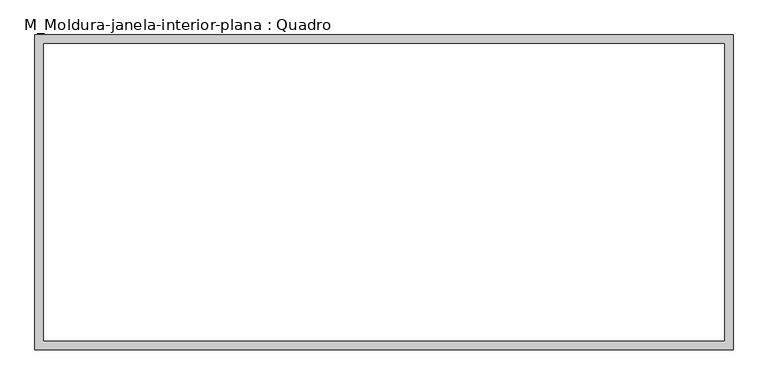
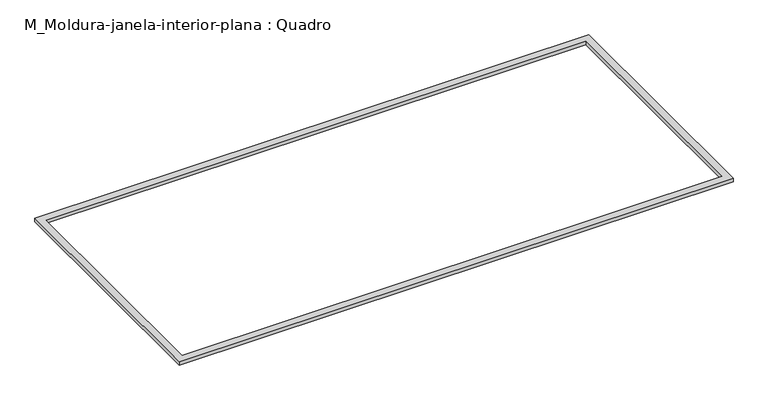
"""IFC4 building model written with IfcOpenShell, lengths in millimetres: proxy geometry, M_Moldura-janela-interior-plana : Quadro."""

import ifcopenshell
import ifcopenshell.guid

model = None  # the IFC model being written
_history = None  # IfcOwnerHistory: only IFC2X3 demands one
_inside = {}  # id of a spatial element -> (the spatial element, [elements in it])
_under = {}  # id of a project, library or spatial element -> (it, [spatial elements below it])
_declared = {}  # id of a project -> (the project, [libraries it declares])
_typed = {}  # id of a type object -> (the type object, [elements of that type])
_made_of = {}  # id of a material, layer set ... -> (it, [elements and type objects made of it])


def new_model(schema):
    """Start an empty IFC model of exactly this schema.

    Asked for "IFC4X3", IfcOpenShell would pick the latest addendum, in which some entities
    have other attributes; the version numbers below select the first issue.
    IFC2X3 requires an IfcOwnerHistory on every rooted entity: one is made here for all.
    """
    global model, _history
    if schema == "IFC4X3":
        model = ifcopenshell.file(schema_version=(4, 3, 0, 0))
    else:
        model = ifcopenshell.file(schema=schema)
    _inside.clear()
    _under.clear()
    _declared.clear()
    _typed.clear()
    _made_of.clear()
    _history = None
    if model.schema == "IFC2X3":
        org = make("IfcOrganization", Name="unknown")
        user = make(
            "IfcPersonAndOrganization",
            ThePerson=make("IfcPerson", FamilyName="unknown"),
            TheOrganization=org,
        )
        app = make(
            "IfcApplication",
            ApplicationDeveloper=org,
            Version="unknown",
            ApplicationFullName="unknown",
            ApplicationIdentifier="unknown",
        )
        _history = make(
            "IfcOwnerHistory",
            OwningUser=user,
            OwningApplication=app,
            ChangeAction="ADDED",
            CreationDate=0,
        )
    return model


def make(cls, **values):
    """One entity of the class cls with the attributes given. An attribute that is None is left unset."""
    return model.create_entity(
        cls, **{name: value for name, value in values.items() if value is not None}
    )


def rooted(cls, **values):
    """An entity with a GlobalId (a new one), such as an element, a storey or a relation."""
    return make(cls, GlobalId=ifcopenshell.guid.new(), OwnerHistory=_history, **values)


def si_unit(unit_type, name, prefix=None):
    """IfcSIUnit, for example si_unit("LENGTHUNIT", "METRE", prefix="MILLI")."""
    return make("IfcSIUnit", UnitType=unit_type, Prefix=prefix, Name=name)


def assignment(units):
    """IfcUnitAssignment: the units of a project."""
    return None if units is None else make("IfcUnitAssignment", Units=units)


def point(xyz):
    """IfcCartesianPoint."""
    return None if xyz is None else make("IfcCartesianPoint", Coordinates=xyz)


def direction(xyz):
    """IfcDirection."""
    return None if xyz is None else make("IfcDirection", DirectionRatios=xyz)


def frame(location, z_axis=None, x_axis=None):
    """IfcAxis2Placement3D, a coordinate frame: its origin and axes. An axis left out is left unset."""
    return make(
        "IfcAxis2Placement3D",
        Location=point(location),
        Axis=direction(z_axis),
        RefDirection=direction(x_axis),
    )


def origin():
    """The frame at (0, 0, 0) with its axes left unset."""
    return frame((0.0, 0.0, 0.0))


def origin_with_axes():
    """The frame at (0, 0, 0) with the z axis (0, 0, 1) and the x axis (1, 0, 0) written out."""
    return frame((0.0, 0.0, 0.0), z_axis=(0.0, 0.0, 1.0), x_axis=(1.0, 0.0, 0.0))


def place(relative_to, where):
    """IfcLocalPlacement: puts the frame where relative to a parent placement (None: the world)."""
    return make(
        "IfcLocalPlacement", PlacementRelTo=relative_to, RelativePlacement=where
    )


def context(
    kind, dimensions, precision=None, world=None, true_north=None, identifier=None
):
    """IfcGeometricRepresentationContext, for example the 3D "Model" context."""
    return make(
        "IfcGeometricRepresentationContext",
        ContextIdentifier=identifier,
        ContextType=kind,
        CoordinateSpaceDimension=dimensions,
        Precision=precision,
        WorldCoordinateSystem=world,
        TrueNorth=true_north,
    )


def project(units=None, contexts=None):
    """IfcProject with its units and contexts."""
    return rooted(
        "IfcProject",
        Name="project",
        RepresentationContexts=contexts,
        UnitsInContext=assignment(units),
    )


def spatial(cls, under=None, at=None, **own):
    """A site, building, storey or space (cls), placed at a placement, below another one or the project."""
    s = rooted(cls, ObjectPlacement=at, **own)
    if under is not None:
        _under.setdefault(under.id(), (under, []))[1].append(s)
    return s


def polyline(points):
    """IfcPolyline through the points."""
    return make("IfcPolyline", Points=[point(p) for p in points])


def outline(outer, holes=None, kind="AREA"):
    """IfcArbitraryClosedProfileDef: a profile drawn as a closed curve; with holes, ...WithVoids."""
    if holes is None:
        return make("IfcArbitraryClosedProfileDef", ProfileType=kind, OuterCurve=outer)
    return make(
        "IfcArbitraryProfileDefWithVoids",
        ProfileType=kind,
        OuterCurve=outer,
        InnerCurves=holes,
    )


def extrude(swept, where, along, depth):
    """IfcExtrudedAreaSolid: the profile swept, set in the frame where, extruded along a direction by depth."""
    return make(
        "IfcExtrudedAreaSolid",
        SweptArea=swept,
        Position=where,
        ExtrudedDirection=direction(along),
        Depth=depth,
    )


def shape(context_of_items, identifier, shape_type, items):
    """IfcShapeRepresentation: the items that make up one representation, for example the "Body"."""
    return make(
        "IfcShapeRepresentation",
        ContextOfItems=context_of_items,
        RepresentationIdentifier=identifier,
        RepresentationType=shape_type,
        Items=items,
    )


def source(mapping_origin, context_of_items, identifier, shape_type, items):
    """IfcRepresentationMap: a shape defined once, which mapped items show again and again."""
    return make(
        "IfcRepresentationMap",
        MappingOrigin=mapping_origin,
        MappedRepresentation=shape(context_of_items, identifier, shape_type, items),
    )


def transform(
    local_origin,
    x_axis=None,
    y_axis=None,
    z_axis=None,
    scale=None,
    scale2=None,
    scale3=None,
    uniform=True,
):
    """IfcCartesianTransformationOperator3D, or its non-uniform kind. x_axis, y_axis, z_axis: its Axis1, 2, 3."""
    if uniform:
        return make(
            "IfcCartesianTransformationOperator3D",
            Axis1=direction(x_axis),
            Axis2=direction(y_axis),
            LocalOrigin=point(local_origin),
            Scale=scale,
            Axis3=direction(z_axis),
        )
    return make(
        "IfcCartesianTransformationOperator3DnonUniform",
        Axis1=direction(x_axis),
        Axis2=direction(y_axis),
        LocalOrigin=point(local_origin),
        Scale=scale,
        Axis3=direction(z_axis),
        Scale2=scale2,
        Scale3=scale3,
    )


def mapped(mapping_source, mapping_target):
    """IfcMappedItem: shows the shape of a source again, moved by a transform."""
    return make(
        "IfcMappedItem", MappingSource=mapping_source, MappingTarget=mapping_target
    )


def made_of(thing, what):
    """Note that an element or type object is made of a material, layer set ...; save() writes the relation."""
    if what is not None:
        _made_of.setdefault(what.id(), (what, []))[1].append(thing)
    return thing


def element(
    cls,
    number,
    at=None,
    inside=None,
    cuts=None,
    type_object=None,
    material=None,
    context=None,
    identifier="Body",
    shape_type=None,
    held_by="IfcProductDefinitionShape",
    body=None,
    shapes=None,
    **own,
):
    """One element of the class cls, such as IfcWall. Its Tag is "e" and its number.

    at: its placement. inside: the storey or other place that contains it. cuts: it is an
    opening in that element (IfcRelVoidsElement). A single representation is given by context,
    identifier, shape_type and body (its items); several are given by shapes. held_by: the class
    of the entity that holds the representations. save() writes the other relations.
    """
    e = rooted(cls, Tag="e%d" % number, ObjectPlacement=at, **own)
    if body is not None:
        shapes = [shape(context, identifier, shape_type, body)]
    if shapes is not None:
        e.Representation = make(held_by, Representations=shapes)
    if inside is not None:
        _inside.setdefault(inside.id(), (inside, []))[1].append(e)
    if cuts is not None:
        rooted(
            "IfcRelVoidsElement", RelatingBuildingElement=cuts, RelatedOpeningElement=e
        )
    if type_object is not None:
        _typed.setdefault(type_object.id(), (type_object, []))[1].append(e)
    return made_of(e, material)


def aggregate(whole, parts):
    """IfcRelAggregates: a whole, such as a stair, and the parts it consists of."""
    return rooted("IfcRelAggregates", RelatingObject=whole, RelatedObjects=parts)


def save(model, path):
    """Write the relations noted so far, then the file.

    IfcRelAggregates (storeys below a building ...), IfcRelContainedInSpatialStructure (elements
    in a storey), IfcRelDefinesByType, IfcRelAssociatesMaterial and IfcRelDeclares: one each for
    every whole, place, type object, material and project.
    """
    for whole, parts in _under.values():
        aggregate(whole, parts)
    for where, things in _inside.values():
        rooted(
            "IfcRelContainedInSpatialStructure",
            RelatedElements=things,
            RelatingStructure=where,
        )
    for kind, things in _typed.values():
        rooted("IfcRelDefinesByType", RelatedObjects=things, RelatingType=kind)
    for what, things in _made_of.values():
        rooted("IfcRelAssociatesMaterial", RelatedObjects=things, RelatingMaterial=what)
    for by, libraries in _declared.values():
        rooted("IfcRelDeclares", RelatingContext=by, RelatedDefinitions=libraries)
    model.write(path)


def m_moldura_janela_interior_plana_quadro_7123fc9e(model_context):
    return source(origin(), model_context, "Body", "SweptSolid", [
        extrude(outline(polyline([(2322.3, 47.3), (2322.3, -2047.3), (-2322.3, -2047.3), (-2322.3, 47.3), (2322.3, 47.3)]), holes=[polyline([(2262.3, -12.7), (-2262.3, -12.7), (-2262.3, -1987.3), (2262.3, -1987.3), (2262.3, -12.7)])]), origin_with_axes(), (0.0, 0.0, 1.0), 30.0),
    ])


if __name__ == "__main__":
    model = new_model("IFC4")
    model_context = context("Model", 3, world=origin())
    ifc_project = project(units=[si_unit("LENGTHUNIT", "METRE", prefix="MILLI")], contexts=[model_context])
    site = spatial("IfcSite", under=ifc_project)
    building = spatial("IfcBuilding", under=site)
    placement = place(None, origin())
    m_moldura_janela_interior_plana_quadro_shape = m_moldura_janela_interior_plana_quadro_7123fc9e(model_context)
    element("IfcBuildingElementProxy", 1, Name="M_Moldura-janela-interior-plana : Quadro", ObjectType="M_Moldura-janela-interior-plana : Quadro", at=placement, inside=building, context=model_context, shape_type="MappedRepresentation", body=[
        mapped(m_moldura_janela_interior_plana_quadro_shape, transform((0.0, 0.0, 0.0), x_axis=(1.0, 0.0, 0.0), y_axis=(0.0, 1.0, 0.0), z_axis=(0.0, 0.0, 1.0))),
    ])
    save(model, "model.ifc")

# Revit data of these elements
# Type "M_Moldura-janela-interior-plana : Quadro"
#   Espessura da apara_Quadro = 0.030 m
#   Largura da apara = 0.060 m
#   Espessura da apara_com peitoril = 0.020 m
#   Espessura do peitoril = 0.030 m
#   Largura da abertura [instance default] = 0.600 m
#   Altura da abertura [instance default] = 0.900 m
#   Default Elevation = 1.200 m
#   Peitoril = no
#   Quadro = yes
#   Material da apara [instance default] = none
# Element 1 (IfcBuildingElementProxy, "M_Moldura-janela-interior-plana : Quadro")
#   Largura da abertura = 4.550 m
#   Altura da abertura = 2.000 m
#   Material da apara = Madeira – Manchada
#   Materials on its faces: "Madeira – Manchada"
# Materials
#   "Madeira – Manchada": class "Madeira", colour RGB 224 178 126, transparency 0, Cost = 0
